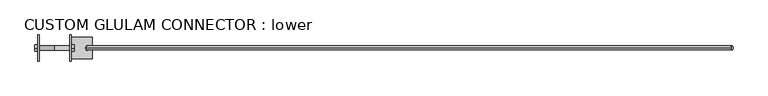
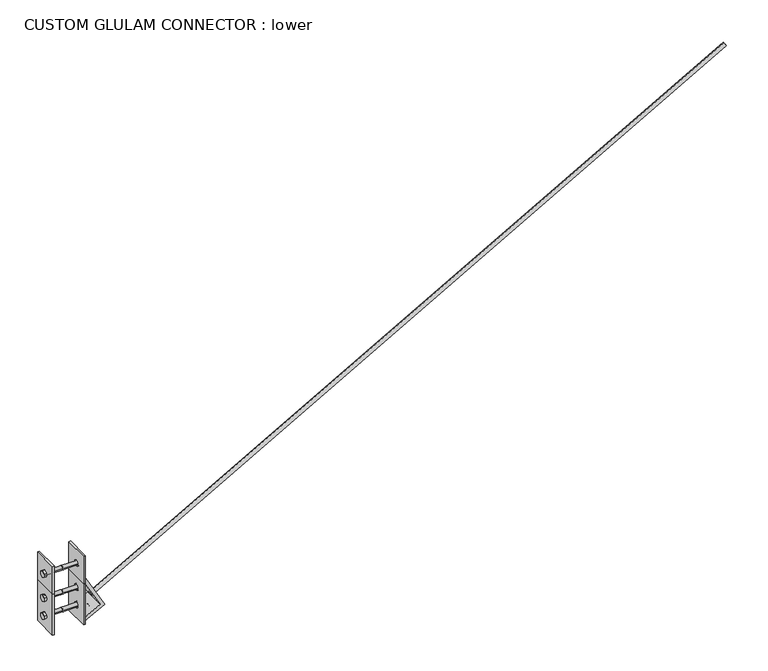
"""IFC4 building model written with IfcOpenShell, lengths in millimetres: fastener geometry, CUSTOM GLULAM CONNECTOR : lower."""

from ifc_helpers import new_model, si_unit, point, frame, frame_2d, origin, place, context, project, spatial, polyline, circle_curve, trimmed, segment, composite_curve, outline, extrude, source, transform, mapped, element, save
from ifc_brep_helpers import plane_surface, revolved_surface, advanced_brep


def custom_glulam_connector_lower_d158587f(model_context):
    return source(origin(), model_context, "Body", "SolidModel", [
        advanced_brep(
        [(-77.7875, 60.325, 211.1375), (-77.7875, 60.325, 7.9375), (-77.7875, 52.3875, 7.9375), (-77.7875, -60.325, 7.9375), (-77.7875, -60.325, 211.1375), (-77.7875, 52.3875, 211.1375), (-77.7875, 13.890625, 160.3375), (-77.7875, -13.890625, 160.3375), (-77.7875, 13.890625, 71.4375), (-77.7875, -13.890625, 71.4375), (-69.85, -13.890625, 160.3375), (-69.85, 13.890625, 160.3375), (-69.85, 13.890625, 71.4375), (-69.85, -13.890625, 71.4375), (-69.85, 60.325, 211.1375), (-69.85, -60.325, 211.1375), (-69.85, -60.325, 7.9375), (-69.85, 60.325, 7.9375)],
        [
            (0, 1),
            (1, 2),
            (2, 3),
            (3, 4),
            (4, 5),
            (5, 0),
            (6, 7, circle_curve(frame((-77.7875, 0.0, 160.3375), z_axis=(1.0, 0.0, 0.0), x_axis=(0.0, 1.0, 0.0)), 13.890625)),
            (7, 6, circle_curve(frame((-77.7875, 0.0, 160.3375), z_axis=(1.0, 0.0, 0.0), x_axis=(0.0, 1.0, 0.0)), 13.890625)),
            (8, 9, circle_curve(frame((-77.7875, 0.0, 71.4375), z_axis=(1.0, 0.0, 0.0), x_axis=(0.0, 1.0, 0.0)), 13.890625)),
            (9, 8, circle_curve(frame((-77.7875, 0.0, 71.4375), z_axis=(1.0, 0.0, 0.0), x_axis=(0.0, 1.0, 0.0)), 13.890625)),
            (10, 11, circle_curve(frame((-69.85, 0.0, 160.3375), z_axis=(1.0, 0.0, 0.0), x_axis=(0.0, 1.0, 0.0)), 13.890625)),
            (11, 6),
            (7, 10),
            (11, 10, circle_curve(frame((-69.85, 0.0, 160.3375), z_axis=(1.0, 0.0, 0.0), x_axis=(0.0, 1.0, 0.0)), 13.890625)),
            (8, 12),
            (12, 13, circle_curve(frame((-69.85, 0.0, 71.4375), z_axis=(1.0, 0.0, 0.0), x_axis=(0.0, 1.0, 0.0)), 13.890625)),
            (13, 9),
            (13, 12, circle_curve(frame((-69.85, 0.0, 71.4375), z_axis=(1.0, 0.0, 0.0), x_axis=(0.0, 1.0, 0.0)), 13.890625)),
            (14, 15),
            (15, 16),
            (16, 17),
            (17, 14),
            (4, 15),
            (14, 0),
            (3, 16),
            (1, 17),
        ],
        [
            plane_surface(frame((-77.7875, -60.325, 211.1375), z_axis=(-1.0, 0.0, 0.0), x_axis=(0.0, -1.0, 0.0))),
            revolved_surface(polyline([(-77.7875, 13.890625, 160.3375), (-69.85, 13.890625, 160.3375)]), (-69.85, 0.0, 160.3375), (-1.0, 0.0, 0.0)),
            revolved_surface(polyline([(-77.7875, 13.890625, 71.4375), (-69.85, 13.890625, 71.4375)]), (-69.85, 0.0, 71.4375), (-1.0, 0.0, 0.0)),
            plane_surface(frame((-69.85, -60.325, 211.1375), z_axis=(1.0, 0.0, 0.0), x_axis=(0.0, 1.0, 0.0))),
            plane_surface(frame((-77.7875, 60.325, 211.1375), z_axis=(0.0, 0.0, 1.0), x_axis=(1.0, 0.0, 0.0))),
            plane_surface(frame((-77.7875, -60.325, 211.1375), z_axis=(0.0, -1.0, 0.0), x_axis=(1.0, 0.0, 0.0))),
            plane_surface(frame((-77.7875, -60.325, 7.9375), z_axis=(0.0, 0.0, -1.0), x_axis=(1.0, 0.0, 0.0))),
            plane_surface(frame((-77.7875, 60.325, 7.9375), z_axis=(0.0, 1.0, 0.0), x_axis=(1.0, 0.0, 0.0))),
        ],
        [
            (0, [[1, 2, 3, 4, 5, 6], [7, 8], [9, 10]]),
            (1, [[11, 12, -8, 13]]),
            (1, [[-7, -12, 14, -13]]),
            (2, [[-9, 15, 16, 17]]),
            (2, [[18, -15, -10, -17]]),
            (3, [[19, 20, 21, 22], [-14, -11], [-16, -18]]),
            (4, [[23, -19, 24, -6, -5]]),
            (5, [[25, -20, -23, -4]]),
            (6, [[26, -21, -25, -3, -2]]),
            (7, [[-24, -22, -26, -1]]),
        ],
    ),
        extrude(outline(polyline([(-14.2875, 168.586392), (0.0, 176.8352839), (14.2875, 168.586392), (14.2875, 152.088608), (0.0, 143.8397161), (-14.2875, 152.088608), (-14.2875, 168.586392)])), frame((-90.4875, 0.0, 0.0), z_axis=(1.0, 0.0, 0.0), x_axis=(0.0, 1.0, 0.0)), (0.0, 0.0, 1.0), 12.7),
        extrude(outline(composite_curve([segment(trimmed(circle_curve(frame_2d((0.0, 160.3375)), 9.525), [point((-9.525, 160.3375))], [point((9.525, 160.3375))], False, "CARTESIAN"), True, "CONTINUOUS"), segment(trimmed(circle_curve(frame_2d((0.0, 160.3375)), 9.525), [point((9.525, 160.3375))], [point((-9.525, 160.3375))], False, "CARTESIAN"), True, "CONTINUOUS")], self_intersect=False)), frame((-77.7875, 0.0, 0.0), z_axis=(1.0, 0.0, 0.0), x_axis=(0.0, 1.0, 0.0)), (0.0, 0.0, 1.0), 76.2),
        extrude(outline(polyline([(-14.2875, 79.686392), (0.0, 87.9352839), (14.2875, 79.686392), (14.2875, 63.188608), (0.0, 54.9397161), (-14.2875, 63.188608), (-14.2875, 79.686392)])), frame((-90.4875, 0.0, 0.0), z_axis=(1.0, 0.0, 0.0), x_axis=(0.0, 1.0, 0.0)), (0.0, 0.0, 1.0), 12.7),
        extrude(outline(composite_curve([segment(trimmed(circle_curve(frame_2d((0.0, 71.4375)), 9.525), [point((-9.525, 71.4375))], [point((9.525, 71.4375))], False, "CARTESIAN"), True, "CONTINUOUS"), segment(trimmed(circle_curve(frame_2d((0.0, 71.4375)), 9.525), [point((9.525, 71.4375))], [point((-9.525, 71.4375))], False, "CARTESIAN"), True, "CONTINUOUS")], self_intersect=False)), frame((-77.7875, 0.0, 0.0), z_axis=(1.0, 0.0, 0.0), x_axis=(0.0, 1.0, 0.0)), (0.0, 0.0, 1.0), 76.2),
        extrude(outline(polyline([(-14.2875, 168.586392), (0.0, 176.8352839), (14.2875, 168.586392), (14.2875, 152.088608), (0.0, 143.8397161), (-14.2875, 152.088608), (-14.2875, 168.586392)])), frame((-90.4875, 0.0, 0.0), z_axis=(1.0, 0.0, 0.0), x_axis=(0.0, 1.0, 0.0)), (0.0, 0.0, 1.0), 12.7),
        extrude(outline(composite_curve([segment(trimmed(circle_curve(frame_2d((0.0, 160.3375)), 9.525), [point((-9.525, 160.3375))], [point((9.525, 160.3375))], False, "CARTESIAN"), True, "CONTINUOUS"), segment(trimmed(circle_curve(frame_2d((0.0, 160.3375)), 9.525), [point((9.525, 160.3375))], [point((-9.525, 160.3375))], False, "CARTESIAN"), True, "CONTINUOUS")], self_intersect=False)), frame((-77.7875, 0.0, 0.0), z_axis=(1.0, 0.0, 0.0), x_axis=(0.0, 1.0, 0.0)), (0.0, 0.0, 1.0), 76.2),
        advanced_brep(
        [(77.7875, 60.325, 211.1375), (77.7875, 52.3875, 211.1375), (77.7875, -60.325, 211.1375), (77.7875, -60.325, 7.9375), (77.7875, 52.3875, 7.9375), (77.7875, 60.325, 7.9375), (77.7875, 13.890625, 71.4375), (77.7875, -13.890625, 71.4375), (77.7875, 13.890625, 160.3375), (77.7875, -13.890625, 160.3375), (69.85, -13.890625, 160.3375), (69.85, 13.890625, 160.3375), (69.85, -13.890625, 71.4375), (69.85, 13.890625, 71.4375), (69.85, 60.325, 211.1375), (69.85, 60.325, 7.9375), (69.85, -60.325, 7.9375), (69.85, -60.325, 211.1375)],
        [
            (0, 1),
            (1, 2),
            (2, 3),
            (3, 4),
            (4, 5),
            (5, 0),
            (6, 7, circle_curve(frame((77.7875, 0.0, 71.4375), z_axis=(-1.0, 0.0, 0.0), x_axis=(0.0, 1.0, 0.0)), 13.890625)),
            (7, 6, circle_curve(frame((77.7875, 0.0, 71.4375), z_axis=(-1.0, 0.0, 0.0), x_axis=(0.0, 1.0, 0.0)), 13.890625)),
            (8, 9, circle_curve(frame((77.7875, 0.0, 160.3375), z_axis=(-1.0, 0.0, 0.0), x_axis=(0.0, 1.0, 0.0)), 13.890625)),
            (9, 8, circle_curve(frame((77.7875, 0.0, 160.3375), z_axis=(-1.0, 0.0, 0.0), x_axis=(0.0, 1.0, 0.0)), 13.890625)),
            (10, 9),
            (8, 11),
            (11, 10, circle_curve(frame((69.85, 0.0, 160.3375), z_axis=(-1.0, 0.0, 0.0), x_axis=(0.0, 1.0, 0.0)), 13.890625)),
            (10, 11, circle_curve(frame((69.85, 0.0, 160.3375), z_axis=(-1.0, 0.0, 0.0), x_axis=(0.0, 1.0, 0.0)), 13.890625)),
            (7, 12),
            (12, 13, circle_curve(frame((69.85, 0.0, 71.4375), z_axis=(-1.0, 0.0, 0.0), x_axis=(0.0, 1.0, 0.0)), 13.890625)),
            (13, 6),
            (13, 12, circle_curve(frame((69.85, 0.0, 71.4375), z_axis=(-1.0, 0.0, 0.0), x_axis=(0.0, 1.0, 0.0)), 13.890625)),
            (14, 15),
            (15, 16),
            (16, 17),
            (17, 14),
            (0, 14),
            (17, 2),
            (16, 3),
            (15, 5),
        ],
        [
            plane_surface(frame((77.7875, -60.325, 211.1375), z_axis=(1.0, 0.0, 0.0), x_axis=(0.0, -1.0, 0.0))),
            revolved_surface(polyline([(77.7875, 13.890625, 160.3375), (69.85, 13.890625, 160.3375)]), (69.85, 0.0, 160.3375), (1.0, 0.0, 0.0)),
            revolved_surface(polyline([(77.7875, 13.890625, 71.4375), (69.85, 13.890625, 71.4375)]), (69.85, 0.0, 71.4375), (1.0, 0.0, 0.0)),
            plane_surface(frame((69.85, -60.325, 211.1375), z_axis=(-1.0, 0.0, 0.0), x_axis=(0.0, 1.0, 0.0))),
            plane_surface(frame((77.7875, 60.325, 211.1375), z_axis=(0.0, 0.0, 1.0), x_axis=(-1.0, 0.0, 0.0))),
            plane_surface(frame((77.7875, -60.325, 211.1375), z_axis=(0.0, -1.0, 0.0), x_axis=(-1.0, 0.0, 0.0))),
            plane_surface(frame((77.7875, -60.325, 7.9375), z_axis=(0.0, 0.0, -1.0), x_axis=(-1.0, 0.0, 0.0))),
            plane_surface(frame((77.7875, 60.325, 7.9375), z_axis=(0.0, 1.0, 0.0), x_axis=(-1.0, 0.0, 0.0))),
        ],
        [
            (0, [[1, 2, 3, 4, 5, 6], [7, 8], [9, 10]]),
            (1, [[11, -9, 12, 13]]),
            (1, [[-11, 14, -12, -10]]),
            (2, [[15, 16, 17, -8]]),
            (2, [[-15, -7, -17, 18]]),
            (3, [[19, 20, 21, 22], [-18, -16], [-13, -14]]),
            (4, [[-2, -1, 23, -22, 24]]),
            (5, [[-3, -24, -21, 25]]),
            (6, [[-5, -4, -25, -20, 26]]),
            (7, [[-6, -26, -19, -23]]),
        ],
    ),
        extrude(outline(polyline([(-14.2875, 168.586392), (0.0, 176.8352839), (14.2875, 168.586392), (14.2875, 152.088608), (0.0, 143.8397161), (-14.2875, 152.088608), (-14.2875, 168.586392)])), frame((77.7875, 0.0, 0.0), z_axis=(1.0, 0.0, 0.0), x_axis=(0.0, 1.0, 0.0)), (0.0, 0.0, 1.0), 12.7),
        extrude(outline(composite_curve([segment(trimmed(circle_curve(frame_2d((0.0, 160.3375)), 9.525), [point((-9.525, 160.3375))], [point((9.525, 160.3375))], False, "CARTESIAN"), True, "CONTINUOUS"), segment(trimmed(circle_curve(frame_2d((0.0, 160.3375)), 9.525), [point((9.525, 160.3375))], [point((-9.525, 160.3375))], False, "CARTESIAN"), True, "CONTINUOUS")], self_intersect=False)), frame((1.5875, 0.0, 0.0), z_axis=(1.0, 0.0, 0.0), x_axis=(0.0, 1.0, 0.0)), (0.0, 0.0, 1.0), 76.2),
        extrude(outline(polyline([(-14.2875, 79.686392), (0.0, 87.9352839), (14.2875, 79.686392), (14.2875, 63.188608), (0.0, 54.9397161), (-14.2875, 63.188608), (-14.2875, 79.686392)])), frame((77.7875, 0.0, 0.0), z_axis=(1.0, 0.0, 0.0), x_axis=(0.0, 1.0, 0.0)), (0.0, 0.0, 1.0), 12.7),
        extrude(outline(composite_curve([segment(trimmed(circle_curve(frame_2d((0.0, 71.4375)), 9.525), [point((-9.525, 71.4375))], [point((9.525, 71.4375))], False, "CARTESIAN"), True, "CONTINUOUS"), segment(trimmed(circle_curve(frame_2d((0.0, 71.4375)), 9.525), [point((9.525, 71.4375))], [point((-9.525, 71.4375))], False, "CARTESIAN"), True, "CONTINUOUS")], self_intersect=False)), frame((1.5875, 0.0, 0.0), z_axis=(1.0, 0.0, 0.0), x_axis=(0.0, 1.0, 0.0)), (0.0, 0.0, 1.0), 76.2),
        extrude(outline(polyline([(-14.2875, 168.586392), (0.0, 176.8352839), (14.2875, 168.586392), (14.2875, 152.088608), (0.0, 143.8397161), (-14.2875, 152.088608), (-14.2875, 168.586392)])), frame((77.7875, 0.0, 0.0), z_axis=(1.0, 0.0, 0.0), x_axis=(0.0, 1.0, 0.0)), (0.0, 0.0, 1.0), 12.7),
        extrude(outline(composite_curve([segment(trimmed(circle_curve(frame_2d((0.0, 160.3375)), 9.525), [point((-9.525, 160.3375))], [point((9.525, 160.3375))], False, "CARTESIAN"), True, "CONTINUOUS"), segment(trimmed(circle_curve(frame_2d((0.0, 160.3375)), 9.525), [point((9.525, 160.3375))], [point((-9.525, 160.3375))], False, "CARTESIAN"), True, "CONTINUOUS")], self_intersect=False)), frame((1.5875, 0.0, 0.0), z_axis=(1.0, 0.0, 0.0), x_axis=(0.0, 1.0, 0.0)), (0.0, 0.0, 1.0), 76.2),
        advanced_brep(
        [(-77.7875, 60.325, 350.8375), (-77.7875, 60.325, 211.1375), (-77.7875, -52.3875, 211.1375), (-77.7875, -60.325, 211.1375), (-77.7875, -60.325, 350.8375), (-77.7875, -52.3875, 350.8375), (-77.7875, 13.890625, 280.9875), (-77.7875, -13.890625, 280.9875), (-69.85, 60.325, 350.8375), (-69.85, -60.325, 350.8375), (-69.85, -60.325, 211.1375), (-69.85, 60.325, 211.1375), (-69.85, -13.890625, 280.9875), (-69.85, 13.890625, 280.9875)],
        [
            (0, 1),
            (1, 2),
            (2, 3),
            (3, 4),
            (4, 5),
            (5, 0),
            (6, 7, circle_curve(frame((-77.7875, 0.0, 280.9875), z_axis=(1.0, 0.0, 0.0), x_axis=(0.0, 1.0, 0.0)), 13.890625)),
            (7, 6, circle_curve(frame((-77.7875, 0.0, 280.9875), z_axis=(1.0, 0.0, 0.0), x_axis=(0.0, 1.0, 0.0)), 13.890625)),
            (8, 9),
            (9, 10),
            (10, 11),
            (11, 8),
            (12, 13, circle_curve(frame((-69.85, 0.0, 280.9875), z_axis=(-1.0, 0.0, 0.0), x_axis=(0.0, 1.0, 0.0)), 13.890625)),
            (13, 12, circle_curve(frame((-69.85, 0.0, 280.9875), z_axis=(-1.0, 0.0, 0.0), x_axis=(0.0, 1.0, 0.0)), 13.890625)),
            (4, 9),
            (8, 0),
            (3, 10),
            (1, 11),
            (13, 6),
            (7, 12),
        ],
        [
            plane_surface(frame((-77.7875, -60.325, 350.8375), z_axis=(-1.0, 0.0, 0.0), x_axis=(0.0, -1.0, 0.0))),
            plane_surface(frame((-69.85, -60.325, 350.8375), z_axis=(1.0, 0.0, 0.0), x_axis=(0.0, 1.0, 0.0))),
            plane_surface(frame((-77.7875, 60.325, 350.8375), z_axis=(0.0, 0.0, 1.0), x_axis=(1.0, 0.0, 0.0))),
            plane_surface(frame((-77.7875, -60.325, 350.8375), z_axis=(0.0, -1.0, 0.0), x_axis=(1.0, 0.0, 0.0))),
            plane_surface(frame((-77.7875, -60.325, 211.1375), z_axis=(0.0, 0.0, -1.0), x_axis=(1.0, 0.0, 0.0))),
            plane_surface(frame((-77.7875, 60.325, 211.1375), z_axis=(0.0, 1.0, 0.0), x_axis=(1.0, 0.0, 0.0))),
            revolved_surface(polyline([(-77.7875, 13.890625, 280.9875), (-69.85, 13.890625, 280.9875)]), (-69.85, 0.0, 280.9875), (-1.0, 0.0, 0.0)),
        ],
        [
            (0, [[1, 2, 3, 4, 5, 6], [7, 8]]),
            (1, [[9, 10, 11, 12], [13, 14]]),
            (2, [[15, -9, 16, -6, -5]]),
            (3, [[17, -10, -15, -4]]),
            (4, [[18, -11, -17, -3, -2]]),
            (5, [[-16, -12, -18, -1]]),
            (6, [[-14, 19, -8, 20]]),
            (6, [[-7, -19, -13, -20]]),
        ],
    ),
        extrude(outline(polyline([(-14.2875, 289.236392), (0.0, 297.4852839), (14.2875, 289.236392), (14.2875, 272.738608), (0.0, 264.4897161), (-14.2875, 272.738608), (-14.2875, 289.236392)])), frame((-90.4875, 0.0, 0.0), z_axis=(1.0, 0.0, 0.0), x_axis=(0.0, 1.0, 0.0)), (0.0, 0.0, 1.0), 12.7),
        extrude(outline(composite_curve([segment(trimmed(circle_curve(frame_2d((0.0, 280.9875)), 9.525), [point((-9.525, 280.9875))], [point((9.525, 280.9875))], False, "CARTESIAN"), True, "CONTINUOUS"), segment(trimmed(circle_curve(frame_2d((0.0, 280.9875)), 9.525), [point((9.525, 280.9875))], [point((-9.525, 280.9875))], False, "CARTESIAN"), True, "CONTINUOUS")], self_intersect=False)), frame((-77.7875, 0.0, 0.0), z_axis=(1.0, 0.0, 0.0), x_axis=(0.0, 1.0, 0.0)), (0.0, 0.0, 1.0), 76.2),
        advanced_brep(
        [(77.7875, 60.325, 350.8375), (77.7875, -52.3875, 350.8375), (77.7875, -60.325, 350.8375), (77.7875, -60.325, 211.1375), (77.7875, -52.3875, 211.1375), (77.7875, 60.325, 211.1375), (77.7875, 13.890625, 280.9875), (77.7875, -13.890625, 280.9875), (69.85, 60.325, 350.8375), (69.85, 60.325, 211.1375), (69.85, -60.325, 211.1375), (69.85, -60.325, 350.8375), (69.85, -13.890625, 280.9875), (69.85, 13.890625, 280.9875)],
        [
            (0, 1),
            (1, 2),
            (2, 3),
            (3, 4),
            (4, 5),
            (5, 0),
            (6, 7, circle_curve(frame((77.7875, 0.0, 280.9875), z_axis=(-1.0, 0.0, 0.0), x_axis=(0.0, 1.0, 0.0)), 13.890625)),
            (7, 6, circle_curve(frame((77.7875, 0.0, 280.9875), z_axis=(-1.0, 0.0, 0.0), x_axis=(0.0, 1.0, 0.0)), 13.890625)),
            (8, 9),
            (9, 10),
            (10, 11),
            (11, 8),
            (12, 13, circle_curve(frame((69.85, 0.0, 280.9875), z_axis=(1.0, 0.0, 0.0), x_axis=(0.0, 1.0, 0.0)), 13.890625)),
            (13, 12, circle_curve(frame((69.85, 0.0, 280.9875), z_axis=(1.0, 0.0, 0.0), x_axis=(0.0, 1.0, 0.0)), 13.890625)),
            (0, 8),
            (11, 2),
            (10, 3),
            (9, 5),
            (12, 7),
            (6, 13),
        ],
        [
            plane_surface(frame((77.7875, -60.325, 350.8375), z_axis=(1.0, 0.0, 0.0), x_axis=(0.0, -1.0, 0.0))),
            plane_surface(frame((69.85, -60.325, 350.8375), z_axis=(-1.0, 0.0, 0.0), x_axis=(0.0, 1.0, 0.0))),
            plane_surface(frame((77.7875, 60.325, 350.8375), z_axis=(0.0, 0.0, 1.0), x_axis=(-1.0, 0.0, 0.0))),
            plane_surface(frame((77.7875, -60.325, 350.8375), z_axis=(0.0, -1.0, 0.0), x_axis=(-1.0, 0.0, 0.0))),
            plane_surface(frame((77.7875, -60.325, 211.1375), z_axis=(0.0, 0.0, -1.0), x_axis=(-1.0, 0.0, 0.0))),
            plane_surface(frame((77.7875, 60.325, 211.1375), z_axis=(0.0, 1.0, 0.0), x_axis=(-1.0, 0.0, 0.0))),
            revolved_surface(polyline([(77.7875, 13.890625, 280.9875), (69.85, 13.890625, 280.9875)]), (69.85, 0.0, 280.9875), (1.0, 0.0, 0.0)),
        ],
        [
            (0, [[1, 2, 3, 4, 5, 6], [7, 8]]),
            (1, [[9, 10, 11, 12], [13, 14]]),
            (2, [[-2, -1, 15, -12, 16]]),
            (3, [[-3, -16, -11, 17]]),
            (4, [[-5, -4, -17, -10, 18]]),
            (5, [[-6, -18, -9, -15]]),
            (6, [[19, -7, 20, -13]]),
            (6, [[-19, -14, -20, -8]]),
        ],
    ),
        extrude(outline(polyline([(-14.2875, 289.236392), (0.0, 297.4852839), (14.2875, 289.236392), (14.2875, 272.738608), (0.0, 264.4897161), (-14.2875, 272.738608), (-14.2875, 289.236392)])), frame((77.7875, 0.0, 0.0), z_axis=(1.0, 0.0, 0.0), x_axis=(0.0, 1.0, 0.0)), (0.0, 0.0, 1.0), 12.7),
        extrude(outline(composite_curve([segment(trimmed(circle_curve(frame_2d((0.0, 280.9875)), 9.525), [point((-9.525, 280.9875))], [point((9.525, 280.9875))], False, "CARTESIAN"), True, "CONTINUOUS"), segment(trimmed(circle_curve(frame_2d((0.0, 280.9875)), 9.525), [point((9.525, 280.9875))], [point((-9.525, 280.9875))], False, "CARTESIAN"), True, "CONTINUOUS")], self_intersect=False)), frame((1.5875, 0.0, 0.0), z_axis=(1.0, 0.0, 0.0), x_axis=(0.0, 1.0, 0.0)), (0.0, 0.0, 1.0), 76.2),
        extrude(outline(composite_curve([segment(trimmed(circle_curve(frame_2d((0.0, -9.525)), 9.525), [point((0.0, -19.05))], [point((0.0, 0.0))], False, "CARTESIAN"), True, "CONTINUOUS"), segment(trimmed(circle_curve(frame_2d((0.0, -9.525)), 9.525), [point((0.0, 0.0))], [point((0.0, -19.05))], False, "CARTESIAN"), True, "CONTINUOUS")], self_intersect=False)), frame((155.1212692, 0.0, 104.8231986), z_axis=(0.8703556959399006, 0.0, 0.4924235601034656), x_axis=(0.0, -1.0, 0.0)), (0.0, 0.0, 1.0), 3429.0),
        advanced_brep(
        [(175.4460516, -50.8, 68.8992672), (77.7875, -50.8, 241.5101729), (77.7875, -50.8, 209.2716667), (153.67429, -50.8, 75.1422194), (77.7875, -50.8, 33.9390543), (77.7875, -50.8, 15.875), (175.4460516, 50.8, 68.8992672), (77.7875, 50.8, 15.875), (77.7875, 50.8, 33.9390543), (153.67429, 50.8, 75.1422194), (77.7875, 50.8, 209.2716667), (77.7875, 50.8, 241.5101729), (155.707561, 0.0, 103.7869313), (145.1543086, 0.0, 122.4397418), (131.3374119, 0.0, 114.6225178), (141.8906643, 0.0, 95.9697073), (123.5760275, 0.0, 58.8001963), (122.8784665, 0.0, 58.4214515), (130.4533618, 0.0, 44.4702298), (131.1509229, 0.0, 44.8489746)],
        [
            (0, 1),
            (1, 2),
            (2, 3),
            (3, 4),
            (4, 5),
            (5, 0),
            (6, 7),
            (7, 8),
            (8, 9),
            (9, 10),
            (10, 11),
            (11, 6),
            (0, 6),
            (11, 1),
            (12, 13, circle_curve(frame((150.4309348, 0.0, 113.1133366), z_axis=(-0.8703556959399006, 0.0, -0.4924235601034656), x_axis=(-0.4924235601034656, 0.0, 0.8703556959399006)), 10.715625)),
            (13, 12, circle_curve(frame((150.4309348, 0.0, 113.1133366), z_axis=(-0.8703556959399006, 0.0, -0.4924235601034656), x_axis=(-0.4924235601034656, 0.0, 0.8703556959399006)), 10.715625)),
            (10, 2),
            (9, 3),
            (14, 15, circle_curve(frame((136.6140381, 0.0, 105.2961126), z_axis=(0.8703556959399006, 0.0, 0.4924235601034656), x_axis=(-0.4924235601034656, 0.0, 0.8703556959399006)), 10.715625)),
            (15, 14, circle_curve(frame((136.6140381, 0.0, 105.2961126), z_axis=(0.8703556959399006, 0.0, 0.4924235601034656), x_axis=(-0.4924235601034656, 0.0, 0.8703556959399006)), 10.715625)),
            (8, 4),
            (16, 17, circle_curve(frame((123.227247, 0.0, 58.6108239), z_axis=(0.47715876025960574, 0.0, -0.8788171126619669), x_axis=(0.8788171126619669, 0.0, 0.47715876025960574)), 0.396875)),
            (17, 16, circle_curve(frame((123.227247, 0.0, 58.6108239), z_axis=(0.47715876025960574, 0.0, -0.8788171126619669), x_axis=(0.8788171126619669, 0.0, 0.47715876025960574)), 0.396875)),
            (7, 5),
            (18, 19, circle_curve(frame((130.8021423, 0.0, 44.6596022), z_axis=(-0.47715876025960574, 0.0, 0.8788171126619669), x_axis=(0.8788171126619669, 0.0, 0.47715876025960574)), 0.396875)),
            (19, 18, circle_curve(frame((130.8021423, 0.0, 44.6596022), z_axis=(-0.47715876025960574, 0.0, 0.8788171126619669), x_axis=(0.8788171126619669, 0.0, 0.47715876025960574)), 0.396875)),
            (12, 15),
            (14, 13),
            (18, 17),
            (16, 19),
        ],
        [
            plane_surface(frame((77.7875, -50.8, 241.5101729), z_axis=(0.0, -1.0, 0.0), x_axis=(-0.4924235601034656, 0.0, 0.8703556959399006))),
            plane_surface(frame((77.7875, 50.8, 241.5101729), z_axis=(0.0, 1.0, 0.0), x_axis=(0.4924235601034656, 0.0, -0.8703556959399006))),
            plane_surface(frame((175.4460516, -50.8, 68.8992672), z_axis=(0.8703556959399006, 0.0, 0.4924235601034656), x_axis=(0.0, 1.0, 0.0))),
            plane_surface(frame((77.7875, -50.8, 241.5101729), z_axis=(-1.0, 0.0, 0.0), x_axis=(0.0, 1.0, 0.0))),
            plane_surface(frame((77.7875, -50.8, 209.2716667), z_axis=(-0.8703556959399004, 0.0, -0.49242356010346605), x_axis=(0.0, 1.0, 0.0))),
            plane_surface(frame((153.67429, -50.8, 75.1422194), z_axis=(-0.4771587602596049, 0.0, 0.8788171126619673), x_axis=(0.0, 1.0, 0.0))),
            plane_surface(frame((77.7875, -50.8, 33.9390543), z_axis=(-1.0, 0.0, 0.0), x_axis=(0.0, 1.0, 0.0))),
            plane_surface(frame((77.7875, -50.8, 15.875), z_axis=(0.47715876025960613, 0.0, -0.8788171126619666), x_axis=(0.0, 1.0, 0.0))),
            revolved_surface(polyline([(131.33741187434143, 0.0, 114.62251781425239), (145.1543085887663, 0.0, 122.43974185430599)]), (150.4309348, 0.0, 113.1133366), (-0.8703556959399006, 0.0, -0.4924235601034656)),
            revolved_surface(polyline([(123.57602749491133, 0.0, 58.80019629723708), (131.15092285819438, 0.0, 44.848974552392434)]), (130.8021423, 0.0, 44.6596022), (-0.47715876025960574, 0.0, 0.8788171126619669)),
        ],
        [
            (0, [[1, 2, 3, 4, 5, 6]]),
            (1, [[7, 8, 9, 10, 11, 12]]),
            (2, [[-1, 13, -12, 14], [15, 16]]),
            (3, [[-2, -14, -11, 17]]),
            (4, [[-3, -17, -10, 18], [19, 20]]),
            (5, [[-4, -18, -9, 21], [22, 23]]),
            (6, [[-5, -21, -8, 24]]),
            (7, [[-6, -24, -7, -13], [25, 26]]),
            (8, [[27, -19, 28, -15]]),
            (8, [[-27, -16, -28, -20]]),
            (9, [[29, -22, 30, -25]]),
            (9, [[-29, -26, -30, -23]]),
        ],
    ),
    ])


if __name__ == "__main__":
    model = new_model("IFC4")
    model_context = context("Model", 3, world=origin())
    ifc_project = project(units=[si_unit("LENGTHUNIT", "METRE", prefix="MILLI")], contexts=[model_context])
    site = spatial("IfcSite", under=ifc_project)
    building = spatial("IfcBuilding", under=site)
    placement = place(None, origin())
    custom_glulam_connector_lower_shape = custom_glulam_connector_lower_d158587f(model_context)
    element("IfcFastener", 1, ObjectType="CUSTOM GLULAM CONNECTOR : lower", at=placement, inside=building, context=model_context, shape_type="MappedRepresentation", body=[
        mapped(custom_glulam_connector_lower_shape, transform((0.0, 0.0, 0.0), x_axis=(1.0, 0.0, 0.0), y_axis=(0.0, 1.0, 0.0), z_axis=(0.0, 0.0, 1.0))),
    ])
    save(model, "model.ifc")

# Revit data of these elements
# Type "CUSTOM GLULAM CONNECTOR : lower"
#   Width - Top = 0' - 5 1/2"
#   Top/Bottom Plate Thickness = 0' - 0 5/16"
#   Top/Bottom Plate - Width = 0' - 7 1/2"
#   Rod Radius = 0' - 0 3/8"
#   Rod Length [instance default] = 11' - 4"
#   Plate Thickness = 0' - 0 5/16"
#   Offset - Upper Plate 2 = 0' - 0"
#   Height of Plate = 0' - 8"
#   Width - Bottom = 0' - 5 1/2"
#   Plate Width = 0' - 4 3/4"
#   Bracket Width = 0' - 4"
#   Bracket Thickness = 0' - 0 5/8"
#   Bracket Offset in X = 0' - 3 1/16"
#   Bracket Offset in Y = 0' - 0 3/8"
#   Bracket Offset = 0' - 0 5/8"
#   Bracket Leg = 0' - 4 3/8"
#   Bracket Hole Radius - Up = 0' - 0 27/64"
#   Bracket Hole Radius - Down = 0' - 0 1/64"
#   Bracket Hole Offset = 0' - 2"
#   Beam Width = 0' - 7 3/8"
#   Angle 2 = 29.50°
#   Angle 1 = 118.50°
#   Top Plate Visible = no
#   Rod Visibility = yes
#   Plate Visibility - Upper Right 2 = no
#   Plate Visibility - Upper Right 1 = yes
#   Plate Visibility - Upper Left 2 = no
#   Plate Visibility - Upper Left 1 = yes
#   Plate Visibility - Lower Right 2 = no
#   Plate Visibility - Lower Right 1 = yes
#   Plate Visibility - Lower Left 2 = no
#   Plate Visibility - Lower Left 1 = yes
#   Bracket Visibility = yes
#   Bottom Plate Visible = no
#   Upper Plates - 2 = element 1407869
#   Upper Plates - 1 = element 1407869
#   Lower Plates = element 1407870
#   Bracket Material = 5/8" STEEL ANGLE (HDG AFTER FABRICATION)
#   URL = ""
# Element 1 (IfcFastener, "CUSTOM GLULAM CONNECTOR : lower")
#   Rod Length = 11' - 3"
#   Materials on its faces: "3/4\" LAG BOLT (THRU BOLT IF PLATE ON OPP. SIDE OF STRUCT MEMBER)", "5/16\" STEEL PLATE (HDG AFTER FABRICATION)", "5/8\" STEEL ANGLE (HDG AFTER FABRICATION)", "3/4\" STEEL ROD (THREADED AT ENDS) - W/ TURN BUCKLE"
# Materials
#   "5/8\" STEEL ANGLE (HDG AFTER FABRICATION)": class "Generic", colour RGB 195 195 195, transparency 0, Cost = 0
#   "3/4\" LAG BOLT (THRU BOLT IF PLATE ON OPP. SIDE OF STRUCT MEMBER)": class "Generic", colour RGB 120 120 120, transparency 0, Cost = 0
#   "5/16\" STEEL PLATE (HDG AFTER FABRICATION)": class "Generic", colour RGB 232 232 232, transparency 0, Cost = 0
#   "3/4\" STEEL ROD (THREADED AT ENDS) - W/ TURN BUCKLE": class "Generic", colour RGB 120 120 120, transparency 0, Cost = 0
